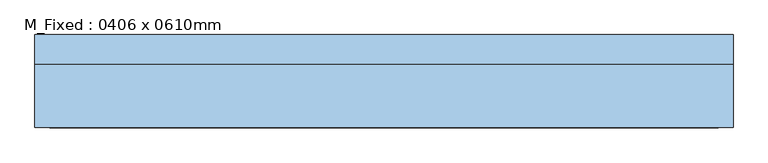
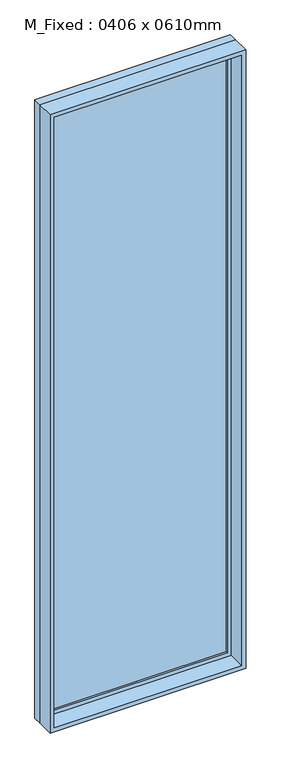
"""IFC4 building model written with IfcOpenShell, lengths in millimetres: window geometry, M_Fixed : 0406 x 0610mm."""

from ifc_helpers import new_model, si_unit, frame, origin, place, context, project, spatial, polyline, outline, extrude, source, transform, mapped, element, save


def m_fixed_0406_x_0610mm_644b55c0(model_context):
    return source(origin(), model_context, "Body", "SweptSolid", [
        extrude(outline(polyline([(-687.0, 78.0), (687.0, 78.0), (687.0, 66.0), (-687.0, 66.0), (-687.0, 78.0)])), frame((0.0, 0.0, 978.0), z_axis=(0.0, 0.0, 1.0), x_axis=(1.0, 0.0, 0.0)), (0.0, 0.0, 1.0), 4874.0),
        extrude(outline(polyline([(5896.0, -731.0), (934.0, -731.0), (934.0, 731.0), (5896.0, 731.0), (5896.0, -731.0)]), holes=[polyline([(5852.0, -687.0), (5852.0, 687.0), (978.0, 687.0), (978.0, -687.0), (5852.0, -687.0)])]), frame((0.0, 50.0, 0.0), z_axis=(0.0, 1.0, 0.0), x_axis=(0.0, 0.0, 1.0)), (0.0, 0.0, 1.0), 44.0),
        extrude(outline(polyline([(5915.0, -750.0), (915.0, -750.0), (915.0, 750.0), (5915.0, 750.0), (5915.0, -750.0)]), holes=[polyline([(5896.0, -731.0), (5896.0, 731.0), (934.0, 731.0), (934.0, -731.0), (5896.0, -731.0)])]), frame((0.0, 50.0, 0.0), z_axis=(0.0, 1.0, 0.0), x_axis=(0.0, 0.0, 1.0)), (0.0, 0.0, 1.0), 63.0),
        extrude(outline(polyline([(5915.0, -750.0), (915.0, -750.0), (915.0, 750.0), (5915.0, 750.0), (5915.0, -750.0)]), holes=[polyline([(5883.0, -718.0), (5883.0, 718.0), (947.0, 718.0), (947.0, -718.0), (5883.0, -718.0)])]), frame((0.0, -87.0, 0.0), z_axis=(0.0, 1.0, 0.0), x_axis=(0.0, 0.0, 1.0)), (0.0, 0.0, 1.0), 137.0),
    ])


if __name__ == "__main__":
    model = new_model("IFC4")
    model_context = context("Model", 3, world=origin())
    ifc_project = project(units=[si_unit("LENGTHUNIT", "METRE", prefix="MILLI")], contexts=[model_context])
    site = spatial("IfcSite", under=ifc_project)
    building = spatial("IfcBuilding", under=site)
    placement = place(None, origin())
    m_fixed_0406_x_0610mm_shape = m_fixed_0406_x_0610mm_644b55c0(model_context)
    element("IfcWindow", 1, ObjectType="M_Fixed : 0406 x 0610mm", at=placement, inside=building, context=model_context, shape_type="MappedRepresentation", body=[
        mapped(m_fixed_0406_x_0610mm_shape, transform((0.0, 0.0, 0.0), x_axis=(1.0, 0.0, 0.0), y_axis=(0.0, 1.0, 0.0), z_axis=(0.0, 0.0, 1.0))),
    ])
    save(model, "model.ifc")

# Revit data of these elements
# Type "M_Fixed : 0406 x 0610mm"
#   Type Mark = "10"
#   Height = 5 m
#   Default Sill Height = 0.915 m
#   Width = 1.5 m
#   Window Inset = 0.019 m
#   Frame Exterior Material = Glass
#   Frame Interior Material = Sash
#   Glass Pane Material = Glass
#   Sash = Sash
#   Wall Closure = (empty or 0)
# Element 1 (IfcWindow, "M_Fixed : 0406 x 0610mm")
#   Materials on its faces: "Sash", "Glass"
# Materials
#   "Glass": class "Glass", colour RGB 218 227 224, transparency 0.85, Description = "Soda Lime Glass", Cost = 0
#   "Sash": class "Wood", colour RGB 136 99 55, transparency 0, Cost = 0
